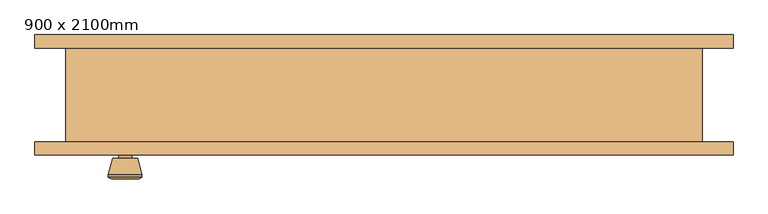
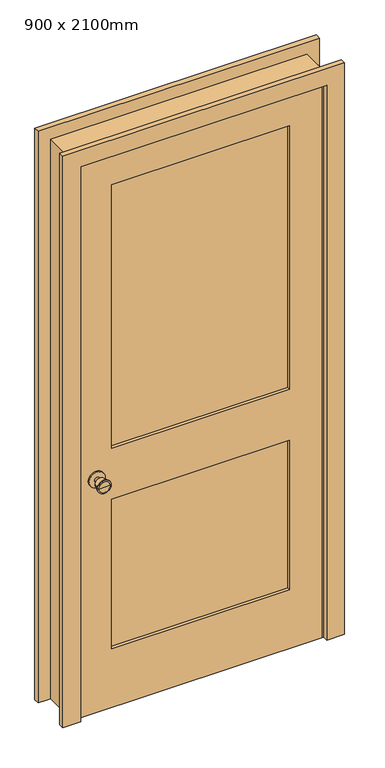
"""IFC4 building model written with IfcOpenShell, lengths in millimetres: door geometry, Porta-Interna-Única-2_Painel-Madeira : 900 x 2100mm."""

from ifc_helpers import new_model, si_unit, point, frame, frame_2d, origin, place, context, project, spatial, polyline, circle_curve, trimmed, segment, composite_curve, outline, extrude, faceted_brep, source, transform, mapped, element, save
from ifc_brep_helpers import plane_surface, cylinder_surface, revolved_surface, advanced_brep


def door_900_x_2100mm_fb9077d6(model_context):
    return source(origin(), model_context, "Body", "SolidModel", [
        advanced_brep(
        [(-386.5, -25.825, 914.4), (-396.5, -25.825, 914.4), (-376.5, -25.825, 914.4), (-366.0241324, 23.175, 914.4), (-406.9758676, 23.175, 914.4), (-386.5, 23.175, 914.4), (-361.5, 21.3471319, 914.4), (-411.5, 21.3471319, 914.4), (-361.5, 17.8834537, 914.4), (-411.5, 17.8834537, 914.4), (-367.863764, -6.825, 914.4), (-405.136236, -6.825, 914.4), (-376.5, -6.825, 914.4), (-396.5, -6.825, 914.4)],
        [
            (0, 1),
            (1, 2, circle_curve(frame((-386.5, -25.825, 914.4), z_axis=(0.0, -1.0, 0.0), x_axis=(-1.0, 0.0, 0.0)), 10.0)),
            (2, 0),
            (2, 1, circle_curve(frame((-386.5, -25.825, 914.4), z_axis=(0.0, -1.0, 0.0), x_axis=(-1.0, 0.0, 0.0)), 10.0)),
            (3, 4, circle_curve(frame((-386.5, 23.175, 914.4), z_axis=(0.0, 1.0, 0.0), x_axis=(-1.0, 0.0, 0.0)), 20.4758676)),
            (4, 5),
            (5, 3),
            (4, 3, circle_curve(frame((-386.5, 23.175, 914.4), z_axis=(0.0, 1.0, 0.0), x_axis=(-1.0, 0.0, 0.0)), 20.4758676)),
            (6, 7, circle_curve(frame((-386.5, 21.3471319, 914.4), z_axis=(0.0, 1.0, 0.0), x_axis=(-1.0, 0.0, 0.0)), 25.0)),
            (7, 4),
            (3, 6),
            (7, 6, circle_curve(frame((-386.5, 21.3471319, 914.4), z_axis=(0.0, 1.0, 0.0), x_axis=(-1.0, 0.0, 0.0)), 25.0)),
            (8, 9, circle_curve(frame((-386.5, 17.8834537, 914.4), z_axis=(0.0, 1.0, 0.0), x_axis=(-1.0, 0.0, 0.0)), 25.0)),
            (9, 7),
            (6, 8),
            (9, 8, circle_curve(frame((-386.5, 17.8834537, 914.4), z_axis=(0.0, 1.0, 0.0), x_axis=(-1.0, 0.0, 0.0)), 25.0)),
            (10, 11, circle_curve(frame((-386.5, -6.825, 914.4), z_axis=(0.0, 1.0, 0.0), x_axis=(-1.0, 0.0, 0.0)), 18.636236)),
            (11, 9),
            (8, 10),
            (11, 10, circle_curve(frame((-386.5, -6.825, 914.4), z_axis=(0.0, 1.0, 0.0), x_axis=(-1.0, 0.0, 0.0)), 18.636236)),
            (12, 13, circle_curve(frame((-386.5, -6.825, 914.4), z_axis=(0.0, 1.0, 0.0), x_axis=(-1.0, 0.0, 0.0)), 10.0)),
            (13, 11),
            (10, 12),
            (13, 12, circle_curve(frame((-386.5, -6.825, 914.4), z_axis=(0.0, 1.0, 0.0), x_axis=(-1.0, 0.0, 0.0)), 10.0)),
            (1, 13),
            (12, 2),
        ],
        [
            plane_surface(frame((-386.5, -25.825, 914.4), z_axis=(0.0, -1.0, 0.0), x_axis=(-1.0, 0.0, 0.0))),
            plane_surface(frame((-386.5, 23.175, 914.4), z_axis=(0.0, 1.0, 0.0), x_axis=(-1.0, 0.0, 0.0))),
            revolved_surface(polyline([(-406.9758676, 23.175, 914.4), (-411.5, 21.3471319, 914.4)]), (-386.5, -25.825, 914.4), (0.0, -1.0, 0.0)),
            cylinder_surface(frame((-386.5, -25.825, 914.4), z_axis=(0.0, -1.0, 0.0), x_axis=(-1.0, 0.0, 0.0)), 25.0),
            revolved_surface(polyline([(-411.5, 17.8834537, 914.4), (-405.136236, -6.825, 914.4)]), (-386.5, -25.825, 914.4), (0.0, -1.0, 0.0)),
            plane_surface(frame((-386.5, -6.825, 914.4), z_axis=(0.0, -1.0, 0.0), x_axis=(-1.0, 0.0, 0.0))),
            cylinder_surface(frame((-386.5, -25.825, 914.4), z_axis=(0.0, -1.0, 0.0), x_axis=(-1.0, 0.0, 0.0)), 10.0),
        ],
        [
            (0, [[1, 2, 3]]),
            (0, [[-3, 4, -1]]),
            (1, [[5, 6, 7]]),
            (1, [[8, -7, -6]]),
            (2, [[9, 10, -5, 11]]),
            (2, [[12, -11, -8, -10]]),
            (3, [[13, 14, -9, 15]]),
            (3, [[16, -15, -12, -14]]),
            (4, [[17, 18, -13, 19]]),
            (4, [[20, -19, -16, -18]]),
            (5, [[21, 22, -17, 23]]),
            (5, [[24, -23, -20, -22]]),
            (6, [[-2, 25, -21, 26]]),
            (6, [[-4, -26, -24, -25]]),
        ],
    ),
        extrude(outline(composite_curve([segment(trimmed(circle_curve(frame_2d((914.4, -386.5)), 30.0), [point((914.4, -416.5))], [point((914.4, -356.5))], False, "CARTESIAN"), True, "CONTINUOUS"), segment(trimmed(circle_curve(frame_2d((914.4, -386.5)), 30.0), [point((914.4, -356.5))], [point((914.4, -416.5))], False, "CARTESIAN"), True, "CONTINUOUS")], self_intersect=False)), frame((0.0, -31.825, 0.0), z_axis=(0.0, 1.0, 0.0), x_axis=(0.0, 0.0, 1.0)), (0.0, 0.0, 1.0), 6.0),
        advanced_brep(
        [(-386.5, -72.825, 914.4), (-376.5, -72.825, 914.4), (-396.5, -72.825, 914.4), (-366.0241324, -121.825, 914.4), (-386.5, -121.825, 914.4), (-406.9758676, -121.825, 914.4), (-361.5, -119.9971319, 914.4), (-411.5, -119.9971319, 914.4), (-361.5, -116.5334537, 914.4), (-411.5, -116.5334537, 914.4), (-367.863764, -91.825, 914.4), (-405.136236, -91.825, 914.4), (-376.5, -91.825, 914.4), (-396.5, -91.825, 914.4)],
        [
            (0, 1),
            (1, 2, circle_curve(frame((-386.5, -72.825, 914.4), z_axis=(0.0, 1.0, 0.0), x_axis=(-1.0, 0.0, 0.0)), 10.0)),
            (2, 0),
            (2, 1, circle_curve(frame((-386.5, -72.825, 914.4), z_axis=(0.0, 1.0, 0.0), x_axis=(-1.0, 0.0, 0.0)), 10.0)),
            (3, 4),
            (4, 5),
            (5, 3, circle_curve(frame((-386.5, -121.825, 914.4), z_axis=(0.0, -1.0, 0.0), x_axis=(-1.0, 0.0, 0.0)), 20.4758676)),
            (3, 5, circle_curve(frame((-386.5, -121.825, 914.4), z_axis=(0.0, -1.0, 0.0), x_axis=(-1.0, 0.0, 0.0)), 20.4758676)),
            (6, 3),
            (5, 7),
            (7, 6, circle_curve(frame((-386.5, -119.9971319, 914.4), z_axis=(0.0, -1.0, 0.0), x_axis=(-1.0, 0.0, 0.0)), 25.0)),
            (6, 7, circle_curve(frame((-386.5, -119.9971319, 914.4), z_axis=(0.0, -1.0, 0.0), x_axis=(-1.0, 0.0, 0.0)), 25.0)),
            (8, 6),
            (7, 9),
            (9, 8, circle_curve(frame((-386.5, -116.5334537, 914.4), z_axis=(0.0, -1.0, 0.0), x_axis=(-1.0, 0.0, 0.0)), 25.0)),
            (8, 9, circle_curve(frame((-386.5, -116.5334537, 914.4), z_axis=(0.0, -1.0, 0.0), x_axis=(-1.0, 0.0, 0.0)), 25.0)),
            (10, 8),
            (9, 11),
            (11, 10, circle_curve(frame((-386.5, -91.825, 914.4), z_axis=(0.0, -1.0, 0.0), x_axis=(-1.0, 0.0, 0.0)), 18.636236)),
            (10, 11, circle_curve(frame((-386.5, -91.825, 914.4), z_axis=(0.0, -1.0, 0.0), x_axis=(-1.0, 0.0, 0.0)), 18.636236)),
            (12, 10),
            (11, 13),
            (13, 12, circle_curve(frame((-386.5, -91.825, 914.4), z_axis=(0.0, -1.0, 0.0), x_axis=(-1.0, 0.0, 0.0)), 10.0)),
            (12, 13, circle_curve(frame((-386.5, -91.825, 914.4), z_axis=(0.0, -1.0, 0.0), x_axis=(-1.0, 0.0, 0.0)), 10.0)),
            (1, 12),
            (13, 2),
        ],
        [
            plane_surface(frame((-386.5, -72.825, 914.4), z_axis=(0.0, 1.0, 0.0), x_axis=(-1.0, 0.0, 0.0))),
            plane_surface(frame((-386.5, -121.825, 914.4), z_axis=(0.0, -1.0, 0.0), x_axis=(-1.0, 0.0, 0.0))),
            revolved_surface(polyline([(-406.9758676, -121.825, 914.4), (-411.5, -119.9971319, 914.4)]), (-386.5, -72.825, 914.4), (0.0, 1.0, 0.0)),
            cylinder_surface(frame((-386.5, -72.825, 914.4), z_axis=(0.0, 1.0, 0.0), x_axis=(-1.0, 0.0, 0.0)), 25.0),
            revolved_surface(polyline([(-411.5, -116.5334537, 914.4), (-405.136236, -91.825, 914.4)]), (-386.5, -72.825, 914.4), (0.0, 1.0, 0.0)),
            plane_surface(frame((-386.5, -91.825, 914.4), z_axis=(0.0, 1.0, 0.0), x_axis=(-1.0, 0.0, 0.0))),
            cylinder_surface(frame((-386.5, -72.825, 914.4), z_axis=(0.0, 1.0, 0.0), x_axis=(-1.0, 0.0, 0.0)), 10.0),
        ],
        [
            (0, [[1, 2, 3]]),
            (0, [[-3, 4, -1]]),
            (1, [[5, 6, 7]]),
            (1, [[-6, -5, 8]]),
            (2, [[9, -7, 10, 11]]),
            (2, [[-10, -8, -9, 12]]),
            (3, [[13, -11, 14, 15]]),
            (3, [[-14, -12, -13, 16]]),
            (4, [[17, -15, 18, 19]]),
            (4, [[-18, -16, -17, 20]]),
            (5, [[21, -19, 22, 23]]),
            (5, [[-22, -20, -21, 24]]),
            (6, [[25, -23, 26, -2]]),
            (6, [[-26, -24, -25, -4]]),
        ],
    ),
        extrude(outline(composite_curve([segment(trimmed(circle_curve(frame_2d((914.4, -386.5)), 30.0), [point((914.4, -416.5))], [point((914.4, -356.5))], False, "CARTESIAN"), True, "CONTINUOUS"), segment(trimmed(circle_curve(frame_2d((914.4, -386.5)), 30.0), [point((914.4, -356.5))], [point((914.4, -416.5))], False, "CARTESIAN"), True, "CONTINUOUS")], self_intersect=False)), frame((0.0, -72.825, 0.0), z_axis=(0.0, 1.0, 0.0), x_axis=(0.0, 0.0, 1.0)), (0.0, 0.0, 1.0), 6.0),
        extrude(outline(polyline([(330.0, -43.4916667), (330.0, -55.1583333), (-330.0, -55.1583333), (-330.0, -43.4916667), (330.0, -43.4916667)])), frame((0.0, 0.0, 1014.4), z_axis=(0.0, 0.0, 1.0), x_axis=(1.0, 0.0, 0.0)), (0.0, 0.0, 1.0), 1030.6),
        extrude(outline(polyline([(330.0, -43.4916667), (330.0, -55.1583333), (-330.0, -55.1583333), (-330.0, -43.4916667), (330.0, -43.4916667)])), frame((0.0, 0.0, 230.0), z_axis=(0.0, 0.0, 1.0), x_axis=(1.0, 0.0, 0.0)), (0.0, 0.0, 1.0), 584.4),
        extrude(outline(polyline([(2165.0, -450.0), (0.0, -450.0), (0.0, 450.0), (2165.0, 450.0), (2165.0, -450.0)]), holes=[polyline([(2045.0, -330.0), (2045.0, 330.0), (1014.4, 330.0), (1014.4, -330.0), (2045.0, -330.0)]), polyline([(814.4, -330.0), (814.4, 330.0), (230.0, 330.0), (230.0, -330.0), (814.4, -330.0)])]), frame((0.0, -66.825, 0.0), z_axis=(0.0, 1.0, 0.0), x_axis=(0.0, 0.0, 1.0)), (0.0, 0.0, 1.0), 35.0),
        faceted_brep([(475.0, -66.825, 0.0), (450.0, -66.825, 0.0), (450.0, -31.825, 0.0), (437.3, -31.825, 0.0), (437.3, 3.1, 0.0), (450.0, 3.1, 0.0), (450.0, 73.175, 0.0), (475.0, 73.175, 0.0), (475.0, 73.175, 2190.0), (475.0, -66.825, 2190.0), (450.0, 73.175, 2165.0), (-450.0, 73.175, 2165.0), (-450.0, 73.175, 0.0), (-475.0, 73.175, 0.0), (-475.0, 73.175, 2190.0), (450.0, 3.1, 2165.0), (437.3, 3.1, 2152.3), (-437.3, 3.1, 2152.3), (-437.3, 3.1, 0.0), (-450.0, 3.1, 0.0), (-450.0, 3.1, 2165.0), (437.3, -31.825, 2152.3), (450.0, -31.825, 2165.0), (-450.0, -31.825, 2165.0), (-450.0, -31.825, 0.0), (-437.3, -31.825, 0.0), (-437.3, -31.825, 2152.3), (450.0, -66.825, 2165.0), (-475.0, -66.825, 2190.0), (-475.0, -66.825, 0.0), (-450.0, -66.825, 0.0), (-450.0, -66.825, 2165.0)], [[[0, 1, 2, 3, 4, 5, 6, 7]], [[7, 8, 9, 0]], [[6, 10, 11, 12, 13, 14, 8, 7]], [[5, 15, 10, 6]], [[4, 16, 17, 18, 19, 20, 15, 5]], [[3, 21, 16, 4]], [[2, 22, 23, 24, 25, 26, 21, 3]], [[1, 27, 22, 2]], [[0, 9, 28, 29, 30, 31, 27, 1]], [[8, 14, 28, 9]], [[15, 20, 11, 10]], [[21, 26, 17, 16]], [[27, 31, 23, 22]], [[29, 13, 12, 19, 18, 25, 24, 30]], [[14, 13, 29, 28]], [[20, 19, 12, 11]], [[26, 25, 18, 17]], [[31, 30, 24, 23]]]),
        extrude(outline(polyline([(0.0, 521.35), (2236.35, 521.35), (2236.35, -521.35), (0.0, -521.35), (0.0, -456.35), (2171.35, -456.35), (2171.35, 456.35), (0.0, 456.35), (0.0, 521.35)])), frame((0.0, 73.175, 0.0), z_axis=(0.0, 1.0, 0.0), x_axis=(0.0, 0.0, 1.0)), (0.0, 0.0, 1.0), 20.0),
        extrude(outline(polyline([(0.0, 521.35), (2236.35, 521.35), (2236.35, -521.35), (0.0, -521.35), (0.0, -456.35), (2171.35, -456.35), (2171.35, 456.35), (0.0, 456.35), (0.0, 521.35)])), frame((0.0, -86.825, 0.0), z_axis=(0.0, 1.0, 0.0), x_axis=(0.0, 0.0, 1.0)), (0.0, 0.0, 1.0), 20.0),
    ])


if __name__ == "__main__":
    model = new_model("IFC4")
    model_context = context("Model", 3, world=origin())
    ifc_project = project(units=[si_unit("LENGTHUNIT", "METRE", prefix="MILLI")], contexts=[model_context])
    site = spatial("IfcSite", under=ifc_project)
    building = spatial("IfcBuilding", under=site)
    placement = place(None, origin())
    door_900_x_2100mm_shape = door_900_x_2100mm_fb9077d6(model_context)
    element("IfcDoor", 1, ObjectType="Porta-Interna-Única-2_Painel-Madeira : 900 x 2100mm", at=placement, inside=building, context=model_context, shape_type="MappedRepresentation", body=[
        mapped(door_900_x_2100mm_shape, transform((0.0, 0.0, 0.0), x_axis=(1.0, 0.0, 0.0), y_axis=(0.0, 1.0, 0.0), z_axis=(0.0, 0.0, 1.0))),
    ])
    save(model, "model.ifc")

# Revit data of these elements
# Type "Porta-Interna-Única-2_Painel-Madeira : 900 x 2100mm"
#   Type Mark = "142"
#   Assembly Code = "C1020300"
#   Analytic Construction = "Madeira"
#   Corrimão superior = 0.120 m
#   Thickness = 0.035 m
#   Thermal Resistance (R) = 0.455703 (m²·K)/W
#   Ângulo de abertura [instance default] = 90.00°
#   Estilos = 0.120 m
#   Rough Width = 0.950 m
#   Rough Height = 2.190 m
#   Bloquear corrimão = 0.200 m
#   Height = 2.165 m
#   Width = 0.900 m
#   Heat Transfer Coefficient (U) = 2.19465 W/(m²·K)
#   Corrimão inferior = 0.230 m
#   Material da apara = Cerejeira
#   Material do painel = Cerejeira
#   Material da moldura = Cerejeira
#   Material da maçaneta = Alumín. 1
#   Visual Light Transmittance = 0
#   Solar Heat Gain Coefficient = 0
#   Wall Closure = (empty or 0)
#   Function = (empty or 0)
# Element 1 (IfcDoor, "Porta-Interna-Única-2_Painel-Madeira : 900 x 2100mm")
#   Materials on its faces: "Cerejeira", "Alumín. 1"
# Materials
#   "Cerejeira": class "Madeira", colour RGB 226 177 128, transparency 0, Description = "Prunus Serotina", Cost = 0
#   "Alumín. 1": class "Metal", colour RGB 247 247 247, transparency 0, Description = "Alumín. 6061", Cost = 0
